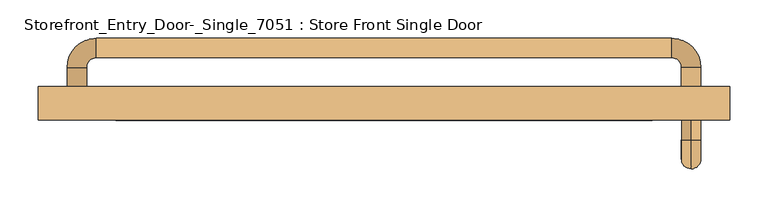
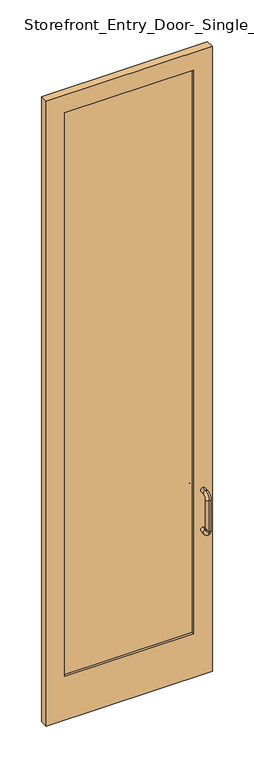
"""IFC4 building model written with IfcOpenShell, lengths in millimetres: door geometry, Storefront_Entry_Door-_Single_7051 : Store Front Single Door."""

import ifcopenshell
import ifcopenshell.guid

model = None  # the IFC model being written
_history = None  # IfcOwnerHistory: only IFC2X3 demands one
_inside = {}  # id of a spatial element -> (the spatial element, [elements in it])
_under = {}  # id of a project, library or spatial element -> (it, [spatial elements below it])
_declared = {}  # id of a project -> (the project, [libraries it declares])
_typed = {}  # id of a type object -> (the type object, [elements of that type])
_made_of = {}  # id of a material, layer set ... -> (it, [elements and type objects made of it])


def new_model(schema):
    """Start an empty IFC model of exactly this schema.

    Asked for "IFC4X3", IfcOpenShell would pick the latest addendum, in which some entities
    have other attributes; the version numbers below select the first issue.
    IFC2X3 requires an IfcOwnerHistory on every rooted entity: one is made here for all.
    """
    global model, _history
    if schema == "IFC4X3":
        model = ifcopenshell.file(schema_version=(4, 3, 0, 0))
    else:
        model = ifcopenshell.file(schema=schema)
    _inside.clear()
    _under.clear()
    _declared.clear()
    _typed.clear()
    _made_of.clear()
    _history = None
    if model.schema == "IFC2X3":
        org = make("IfcOrganization", Name="unknown")
        user = make(
            "IfcPersonAndOrganization",
            ThePerson=make("IfcPerson", FamilyName="unknown"),
            TheOrganization=org,
        )
        app = make(
            "IfcApplication",
            ApplicationDeveloper=org,
            Version="unknown",
            ApplicationFullName="unknown",
            ApplicationIdentifier="unknown",
        )
        _history = make(
            "IfcOwnerHistory",
            OwningUser=user,
            OwningApplication=app,
            ChangeAction="ADDED",
            CreationDate=0,
        )
    return model


def make(cls, **values):
    """One entity of the class cls with the attributes given. An attribute that is None is left unset."""
    return model.create_entity(
        cls, **{name: value for name, value in values.items() if value is not None}
    )


def rooted(cls, **values):
    """An entity with a GlobalId (a new one), such as an element, a storey or a relation."""
    return make(cls, GlobalId=ifcopenshell.guid.new(), OwnerHistory=_history, **values)


def si_unit(unit_type, name, prefix=None):
    """IfcSIUnit, for example si_unit("LENGTHUNIT", "METRE", prefix="MILLI")."""
    return make("IfcSIUnit", UnitType=unit_type, Prefix=prefix, Name=name)


def assignment(units):
    """IfcUnitAssignment: the units of a project."""
    return None if units is None else make("IfcUnitAssignment", Units=units)


def point(xyz):
    """IfcCartesianPoint."""
    return None if xyz is None else make("IfcCartesianPoint", Coordinates=xyz)


def direction(xyz):
    """IfcDirection."""
    return None if xyz is None else make("IfcDirection", DirectionRatios=xyz)


def frame(location, z_axis=None, x_axis=None):
    """IfcAxis2Placement3D, a coordinate frame: its origin and axes. An axis left out is left unset."""
    return make(
        "IfcAxis2Placement3D",
        Location=point(location),
        Axis=direction(z_axis),
        RefDirection=direction(x_axis),
    )


def origin():
    """The frame at (0, 0, 0) with its axes left unset."""
    return frame((0.0, 0.0, 0.0))


def place(relative_to, where):
    """IfcLocalPlacement: puts the frame where relative to a parent placement (None: the world)."""
    return make(
        "IfcLocalPlacement", PlacementRelTo=relative_to, RelativePlacement=where
    )


def context(
    kind, dimensions, precision=None, world=None, true_north=None, identifier=None
):
    """IfcGeometricRepresentationContext, for example the 3D "Model" context."""
    return make(
        "IfcGeometricRepresentationContext",
        ContextIdentifier=identifier,
        ContextType=kind,
        CoordinateSpaceDimension=dimensions,
        Precision=precision,
        WorldCoordinateSystem=world,
        TrueNorth=true_north,
    )


def project(units=None, contexts=None):
    """IfcProject with its units and contexts."""
    return rooted(
        "IfcProject",
        Name="project",
        RepresentationContexts=contexts,
        UnitsInContext=assignment(units),
    )


def spatial(cls, under=None, at=None, **own):
    """A site, building, storey or space (cls), placed at a placement, below another one or the project."""
    s = rooted(cls, ObjectPlacement=at, **own)
    if under is not None:
        _under.setdefault(under.id(), (under, []))[1].append(s)
    return s


def polyline(points):
    """IfcPolyline through the points."""
    return make("IfcPolyline", Points=[point(p) for p in points])


def circle_curve(where, radius):
    """IfcCircle in the frame where."""
    return make("IfcCircle", Position=where, Radius=radius)


def ellipse_curve(where, semi_axis1, semi_axis2):
    """IfcEllipse in the frame where."""
    return make(
        "IfcEllipse", Position=where, SemiAxis1=semi_axis1, SemiAxis2=semi_axis2
    )


def trimmed(basis, trim1, trim2, sense, master):
    """IfcTrimmedCurve: the piece of a basis curve between two trims."""
    return make(
        "IfcTrimmedCurve",
        BasisCurve=basis,
        Trim1=trim1,
        Trim2=trim2,
        SenseAgreement=sense,
        MasterRepresentation=master,
    )


def outline(outer, holes=None, kind="AREA"):
    """IfcArbitraryClosedProfileDef: a profile drawn as a closed curve; with holes, ...WithVoids."""
    if holes is None:
        return make("IfcArbitraryClosedProfileDef", ProfileType=kind, OuterCurve=outer)
    return make(
        "IfcArbitraryProfileDefWithVoids",
        ProfileType=kind,
        OuterCurve=outer,
        InnerCurves=holes,
    )


def extrude(swept, where, along, depth):
    """IfcExtrudedAreaSolid: the profile swept, set in the frame where, extruded along a direction by depth."""
    return make(
        "IfcExtrudedAreaSolid",
        SweptArea=swept,
        Position=where,
        ExtrudedDirection=direction(along),
        Depth=depth,
    )


def shape(context_of_items, identifier, shape_type, items):
    """IfcShapeRepresentation: the items that make up one representation, for example the "Body"."""
    return make(
        "IfcShapeRepresentation",
        ContextOfItems=context_of_items,
        RepresentationIdentifier=identifier,
        RepresentationType=shape_type,
        Items=items,
    )


def source(mapping_origin, context_of_items, identifier, shape_type, items):
    """IfcRepresentationMap: a shape defined once, which mapped items show again and again."""
    return make(
        "IfcRepresentationMap",
        MappingOrigin=mapping_origin,
        MappedRepresentation=shape(context_of_items, identifier, shape_type, items),
    )


def transform(
    local_origin,
    x_axis=None,
    y_axis=None,
    z_axis=None,
    scale=None,
    scale2=None,
    scale3=None,
    uniform=True,
):
    """IfcCartesianTransformationOperator3D, or its non-uniform kind. x_axis, y_axis, z_axis: its Axis1, 2, 3."""
    if uniform:
        return make(
            "IfcCartesianTransformationOperator3D",
            Axis1=direction(x_axis),
            Axis2=direction(y_axis),
            LocalOrigin=point(local_origin),
            Scale=scale,
            Axis3=direction(z_axis),
        )
    return make(
        "IfcCartesianTransformationOperator3DnonUniform",
        Axis1=direction(x_axis),
        Axis2=direction(y_axis),
        LocalOrigin=point(local_origin),
        Scale=scale,
        Axis3=direction(z_axis),
        Scale2=scale2,
        Scale3=scale3,
    )


def mapped(mapping_source, mapping_target):
    """IfcMappedItem: shows the shape of a source again, moved by a transform."""
    return make(
        "IfcMappedItem", MappingSource=mapping_source, MappingTarget=mapping_target
    )


def made_of(thing, what):
    """Note that an element or type object is made of a material, layer set ...; save() writes the relation."""
    if what is not None:
        _made_of.setdefault(what.id(), (what, []))[1].append(thing)
    return thing


def element(
    cls,
    number,
    at=None,
    inside=None,
    cuts=None,
    type_object=None,
    material=None,
    context=None,
    identifier="Body",
    shape_type=None,
    held_by="IfcProductDefinitionShape",
    body=None,
    shapes=None,
    **own,
):
    """One element of the class cls, such as IfcWall. Its Tag is "e" and its number.

    at: its placement. inside: the storey or other place that contains it. cuts: it is an
    opening in that element (IfcRelVoidsElement). A single representation is given by context,
    identifier, shape_type and body (its items); several are given by shapes. held_by: the class
    of the entity that holds the representations. save() writes the other relations.
    """
    e = rooted(cls, Tag="e%d" % number, ObjectPlacement=at, **own)
    if body is not None:
        shapes = [shape(context, identifier, shape_type, body)]
    if shapes is not None:
        e.Representation = make(held_by, Representations=shapes)
    if inside is not None:
        _inside.setdefault(inside.id(), (inside, []))[1].append(e)
    if cuts is not None:
        rooted(
            "IfcRelVoidsElement", RelatingBuildingElement=cuts, RelatedOpeningElement=e
        )
    if type_object is not None:
        _typed.setdefault(type_object.id(), (type_object, []))[1].append(e)
    return made_of(e, material)


def aggregate(whole, parts):
    """IfcRelAggregates: a whole, such as a stair, and the parts it consists of."""
    return rooted("IfcRelAggregates", RelatingObject=whole, RelatedObjects=parts)


def save(model, path):
    """Write the relations noted so far, then the file.

    IfcRelAggregates (storeys below a building ...), IfcRelContainedInSpatialStructure (elements
    in a storey), IfcRelDefinesByType, IfcRelAssociatesMaterial and IfcRelDeclares: one each for
    every whole, place, type object, material and project.
    """
    for whole, parts in _under.values():
        aggregate(whole, parts)
    for where, things in _inside.values():
        rooted(
            "IfcRelContainedInSpatialStructure",
            RelatedElements=things,
            RelatingStructure=where,
        )
    for kind, things in _typed.values():
        rooted("IfcRelDefinesByType", RelatedObjects=things, RelatingType=kind)
    for what, things in _made_of.values():
        rooted("IfcRelAssociatesMaterial", RelatedObjects=things, RelatingMaterial=what)
    for by, libraries in _declared.values():
        rooted("IfcRelDeclares", RelatingContext=by, RelatedDefinitions=libraries)
    model.write(path)


def plane_surface(at):
    """IfcPlane: the flat surface through the origin of the frame at, square to its z axis."""
    return make("IfcPlane", Position=at)


def cylinder_surface(at, radius):
    """IfcCylindricalSurface: all points at the distance radius from the z axis of the frame at."""
    return make("IfcCylindricalSurface", Position=at, Radius=radius)


def revolved_surface(curve, axis_point, axis_direction):
    """IfcSurfaceOfRevolution: the curve turned about the line through axis_point along axis_direction."""
    return make(
        "IfcSurfaceOfRevolution",
        SweptCurve=make("IfcArbitraryOpenProfileDef", ProfileType="CURVE", Curve=curve),
        AxisPosition=make("IfcAxis1Placement", Location=point(axis_point), Axis=direction(axis_direction)),
    )


def advanced_brep(points, edges, surfaces, faces):
    """IfcAdvancedBrep: a solid bounded by faces that lie on surfaces and meet in shared edges.

    An edge is (start, end): straight between two places in points (the first is 0);
    or (start, end, curve); or (start, end, curve, False) where it runs against its curve.
    A face is (place in surfaces, loops), or (place, loops, False) where it looks against
    its surface's normal. A loop lists edges by number (the first is 1), with a minus sign
    where the edge is run from its end to its start. The first loop is the outer one.
    """
    corners = [point(p) for p in points]
    vertices = [make("IfcVertexPoint", VertexGeometry=c) for c in corners]
    made = []
    for start, end, *more in edges:
        made.append(
            make(
                "IfcEdgeCurve",
                EdgeStart=vertices[start],
                EdgeEnd=vertices[end],
                EdgeGeometry=more[0] if more else make("IfcPolyline", Points=[corners[start], corners[end]]),
                SameSense=more[1] if len(more) > 1 else True,
            )
        )
    hull = []
    for where, loops, *sense in faces:
        bounds = []
        for j, loop in enumerate(loops):
            ring = [make("IfcOrientedEdge", EdgeElement=made[abs(k) - 1], Orientation=k > 0) for k in loop]
            bounds.append(
                make(
                    "IfcFaceOuterBound" if j == 0 else "IfcFaceBound",
                    Bound=make("IfcEdgeLoop", EdgeList=ring),
                    Orientation=True,
                )
            )
        hull.append(make("IfcAdvancedFace", Bounds=bounds, FaceSurface=surfaces[where], SameSense=sense[0] if sense else True))
    return make("IfcAdvancedBrep", Outer=make("IfcClosedShell", CfsFaces=hull))


def storefront_entry_door_single_7051_store_front_single_door_77dde46e(model_context):
    return source(origin(), model_context, "Body", "SolidModel", [
        advanced_brep(
        [(402.7714285, -50.8, 1054.1), (402.7714285, -50.8, 1079.5), (402.7714285, -76.2, 1079.5), (402.7714285, -76.2, 1054.1), (402.7714285, -114.3, 1041.4), (402.7714285, -88.9, 1041.4), (402.7714285, -114.3, 863.6), (402.7714285, -88.9, 863.6), (402.7714285, -76.2, 825.5), (402.7714285, -76.2, 850.9), (402.7714285, -50.8, 850.9), (402.7714285, -50.8, 825.5)],
        [
            (0, 1, circle_curve(frame((402.7714285, -50.8, 1066.8), z_axis=(0.0, 1.0, 0.0), x_axis=(0.0, 0.0, 1.0)), 12.7)),
            (1, 0, circle_curve(frame((402.7714285, -50.8, 1066.8), z_axis=(0.0, 1.0, 0.0), x_axis=(0.0, 0.0, 1.0)), 12.7)),
            (1, 2),
            (2, 3, circle_curve(frame((402.7714285, -76.2, 1066.8), z_axis=(0.0, 1.0, 0.0), x_axis=(0.0, 0.0, 1.0)), 12.7)),
            (3, 0),
            (3, 2, circle_curve(frame((402.7714285, -76.2, 1066.8), z_axis=(0.0, 1.0, 0.0), x_axis=(0.0, 0.0, 1.0)), 12.7)),
            (4, 5, circle_curve(frame((402.7714285, -101.6, 1041.4), z_axis=(0.0, 0.0, 1.0), x_axis=(0.0, -1.0, 0.0)), 12.7)),
            (5, 3, circle_curve(frame((402.7714285, -76.2, 1041.4), z_axis=(-1.0, 0.0, 0.0), x_axis=(0.0, 0.0, 1.0)), 12.7)),
            (2, 4, circle_curve(frame((402.7714285, -76.2, 1041.4), z_axis=(1.0, 0.0, 0.0), x_axis=(0.0, 0.0, 1.0)), 38.1)),
            (5, 4, circle_curve(frame((402.7714285, -101.6, 1041.4), z_axis=(0.0, 0.0, 1.0), x_axis=(0.0, -1.0, 0.0)), 12.7)),
            (4, 6),
            (6, 7, circle_curve(frame((402.7714285, -101.6, 863.6), z_axis=(0.0, 0.0, 1.0), x_axis=(0.0, -1.0, 0.0)), 12.7)),
            (7, 5),
            (7, 6, circle_curve(frame((402.7714285, -101.6, 863.6), z_axis=(0.0, 0.0, 1.0), x_axis=(0.0, -1.0, 0.0)), 12.7)),
            (8, 9, circle_curve(frame((402.7714285, -76.2, 838.2), z_axis=(0.0, -1.0, 0.0), x_axis=(0.0, 0.0, -1.0)), 12.7)),
            (9, 7, circle_curve(frame((402.7714285, -76.2, 863.6), z_axis=(-1.0, 0.0, 0.0), x_axis=(0.0, -1.0, 0.0)), 12.7)),
            (6, 8, circle_curve(frame((402.7714285, -76.2, 863.6), z_axis=(1.0, 0.0, 0.0), x_axis=(0.0, -1.0, 0.0)), 38.1)),
            (9, 8, circle_curve(frame((402.7714285, -76.2, 838.2), z_axis=(0.0, -1.0, 0.0), x_axis=(0.0, 0.0, -1.0)), 12.7)),
            (10, 11, circle_curve(frame((402.7714285, -50.8, 838.2), z_axis=(0.0, 1.0, 0.0), x_axis=(0.0, 0.0, -1.0)), 12.7)),
            (11, 10, circle_curve(frame((402.7714285, -50.8, 838.2), z_axis=(0.0, 1.0, 0.0), x_axis=(0.0, 0.0, -1.0)), 12.7)),
            (8, 11),
            (10, 9),
        ],
        [
            plane_surface(frame((402.7714285, -50.8, 1066.8), z_axis=(0.0, 1.0, 0.0), x_axis=(1.0, 0.0, 0.0))),
            cylinder_surface(frame((402.7714285, -50.8, 1066.8), z_axis=(0.0, 1.0, 0.0), x_axis=(0.0, 0.0, 1.0)), 12.7),
            revolved_surface(trimmed(ellipse_curve(frame((402.7714285, -76.2, 1066.8), z_axis=(0.0, -1.0, 0.0), x_axis=(0.0, 0.0, 1.0)), 12.7, 12.7), [point((402.7714285, -76.2, 1054.1))], [point((402.7714285, -76.2, 1079.5))], True, "CARTESIAN"), (402.7714285, -76.2, 1041.4), (-1.0, 0.0, 0.0)),
            revolved_surface(trimmed(ellipse_curve(frame((402.7714285, -76.2, 1066.8), z_axis=(0.0, -1.0, 0.0), x_axis=(0.0, 0.0, 1.0)), 12.7, 12.7), [point((402.7714285, -76.2, 1079.5))], [point((402.7714285, -76.2, 1054.1))], True, "CARTESIAN"), (402.7714285, -76.2, 1041.4), (-1.0, 0.0, 0.0)),
            cylinder_surface(frame((402.7714285, -101.6, 1041.4), z_axis=(0.0, 0.0, 1.0), x_axis=(0.0, -1.0, 0.0)), 12.7),
            revolved_surface(trimmed(ellipse_curve(frame((402.7714285, -101.6, 863.6), z_axis=(0.0, 0.0, -1.0), x_axis=(0.0, -1.0, 0.0)), 12.7, 12.7), [point((402.7714285, -88.9, 863.6))], [point((402.7714285, -114.3, 863.6))], True, "CARTESIAN"), (402.7714285, -76.2, 863.6), (-1.0, 0.0, 0.0)),
            revolved_surface(trimmed(ellipse_curve(frame((402.7714285, -101.6, 863.6), z_axis=(0.0, 0.0, -1.0), x_axis=(0.0, -1.0, 0.0)), 12.7, 12.7), [point((402.7714285, -114.3, 863.6))], [point((402.7714285, -88.9, 863.6))], True, "CARTESIAN"), (402.7714285, -76.2, 863.6), (-1.0, 0.0, 0.0)),
            plane_surface(frame((402.7714285, -50.8, 838.2), z_axis=(0.0, 1.0, 0.0), x_axis=(1.0, 0.0, 0.0))),
            cylinder_surface(frame((402.7714285, -76.2, 838.2), z_axis=(0.0, -1.0, 0.0), x_axis=(0.0, 0.0, -1.0)), 12.7),
        ],
        [
            (0, [[1, 2]]),
            (1, [[3, 4, 5, -2]]),
            (1, [[-5, 6, -3, -1]]),
            (2, [[7, 8, -4, 9]]),
            (3, [[10, -9, -6, -8]]),
            (4, [[11, 12, 13, -7]]),
            (4, [[-13, 14, -11, -10]]),
            (5, [[15, 16, -12, 17]]),
            (6, [[18, -17, -14, -16]]),
            (7, [[19, 20]]),
            (8, [[21, -19, 22, -15]]),
            (8, [[-22, -20, -21, -18]]),
        ],
    ),
        advanced_brep(
        [(390.0714285, -6.35, 1066.8), (415.4714285, -6.35, 1066.8), (415.4714285, 19.05, 1066.8), (390.0714285, 19.05, 1066.8), (377.3714285, 57.15, 1066.8), (377.3714285, 31.75, 1066.8), (-377.3714285, 57.15, 1066.8), (-377.3714285, 31.75, 1066.8), (-415.4714285, 19.05, 1066.8), (-390.0714285, 19.05, 1066.8), (-390.0714285, -6.35, 1066.8), (-415.4714285, -6.35, 1066.8)],
        [
            (0, 1, circle_curve(frame((402.7714285, -6.35, 1066.8), z_axis=(0.0, -1.0, 0.0), x_axis=(1.0, 0.0, 0.0)), 12.7)),
            (1, 0, circle_curve(frame((402.7714285, -6.35, 1066.8), z_axis=(0.0, -1.0, 0.0), x_axis=(1.0, 0.0, 0.0)), 12.7)),
            (1, 2),
            (2, 3, circle_curve(frame((402.7714285, 19.05, 1066.8), z_axis=(0.0, -1.0, 0.0), x_axis=(1.0, 0.0, 0.0)), 12.7)),
            (3, 0),
            (3, 2, circle_curve(frame((402.7714285, 19.05, 1066.8), z_axis=(0.0, -1.0, 0.0), x_axis=(1.0, 0.0, 0.0)), 12.7)),
            (4, 5, circle_curve(frame((377.3714285, 44.45, 1066.8), z_axis=(1.0, 0.0, 0.0), x_axis=(0.0, 1.0, 0.0)), 12.7)),
            (5, 3, circle_curve(frame((377.3714285, 19.05, 1066.8), z_axis=(0.0, 0.0, -1.0), x_axis=(1.0, 0.0, 0.0)), 12.7)),
            (2, 4, circle_curve(frame((377.3714285, 19.05, 1066.8), z_axis=(0.0, 0.0, 1.0), x_axis=(1.0, 0.0, 0.0)), 38.1)),
            (5, 4, circle_curve(frame((377.3714285, 44.45, 1066.8), z_axis=(1.0, 0.0, 0.0), x_axis=(0.0, 1.0, 0.0)), 12.7)),
            (4, 6),
            (6, 7, circle_curve(frame((-377.3714285, 44.45, 1066.8), z_axis=(1.0, 0.0, 0.0), x_axis=(0.0, 1.0, 0.0)), 12.7)),
            (7, 5),
            (7, 6, circle_curve(frame((-377.3714285, 44.45, 1066.8), z_axis=(1.0, 0.0, 0.0), x_axis=(0.0, 1.0, 0.0)), 12.7)),
            (8, 9, circle_curve(frame((-402.7714285, 19.05, 1066.8), z_axis=(0.0, 1.0, 0.0), x_axis=(-1.0, 0.0, 0.0)), 12.7)),
            (9, 7, circle_curve(frame((-377.3714285, 19.05, 1066.8), z_axis=(0.0, 0.0, -1.0), x_axis=(0.0, 1.0, 0.0)), 12.7)),
            (6, 8, circle_curve(frame((-377.3714285, 19.05, 1066.8), z_axis=(0.0, 0.0, 1.0), x_axis=(0.0, 1.0, 0.0)), 38.1)),
            (9, 8, circle_curve(frame((-402.7714285, 19.05, 1066.8), z_axis=(0.0, 1.0, 0.0), x_axis=(-1.0, 0.0, 0.0)), 12.7)),
            (10, 11, circle_curve(frame((-402.7714285, -6.35, 1066.8), z_axis=(0.0, -1.0, 0.0), x_axis=(-1.0, 0.0, 0.0)), 12.7)),
            (11, 10, circle_curve(frame((-402.7714285, -6.35, 1066.8), z_axis=(0.0, -1.0, 0.0), x_axis=(-1.0, 0.0, 0.0)), 12.7)),
            (8, 11),
            (10, 9),
        ],
        [
            plane_surface(frame((402.7714285, -6.35, 1066.8), z_axis=(0.0, -1.0, 0.0), x_axis=(0.0, 0.0, 1.0))),
            cylinder_surface(frame((402.7714285, -6.35, 1066.8), z_axis=(0.0, -1.0, 0.0), x_axis=(1.0, 0.0, 0.0)), 12.7),
            revolved_surface(trimmed(ellipse_curve(frame((402.7714285, 19.05, 1066.8), z_axis=(0.0, 1.0, 0.0), x_axis=(1.0, 0.0, 0.0)), 12.7, 12.7), [point((390.0714285, 19.05, 1066.8))], [point((415.4714285, 19.05, 1066.8))], True, "CARTESIAN"), (377.3714285, 19.05, 1066.8), (0.0, 0.0, -1.0)),
            revolved_surface(trimmed(ellipse_curve(frame((402.7714285, 19.05, 1066.8), z_axis=(0.0, 1.0, 0.0), x_axis=(1.0, 0.0, 0.0)), 12.7, 12.7), [point((415.4714285, 19.05, 1066.8))], [point((390.0714285, 19.05, 1066.8))], True, "CARTESIAN"), (377.3714285, 19.05, 1066.8), (0.0, 0.0, -1.0)),
            cylinder_surface(frame((377.3714285, 44.45, 1066.8), z_axis=(1.0, 0.0, 0.0), x_axis=(0.0, 1.0, 0.0)), 12.7),
            revolved_surface(trimmed(ellipse_curve(frame((-377.3714285, 44.45, 1066.8), z_axis=(-1.0, 0.0, 0.0), x_axis=(0.0, 1.0, 0.0)), 12.7, 12.7), [point((-377.3714285, 31.75, 1066.8))], [point((-377.3714285, 57.15, 1066.8))], True, "CARTESIAN"), (-377.3714285, 19.05, 1066.8), (0.0, 0.0, -1.0)),
            revolved_surface(trimmed(ellipse_curve(frame((-377.3714285, 44.45, 1066.8), z_axis=(-1.0, 0.0, 0.0), x_axis=(0.0, 1.0, 0.0)), 12.7, 12.7), [point((-377.3714285, 57.15, 1066.8))], [point((-377.3714285, 31.75, 1066.8))], True, "CARTESIAN"), (-377.3714285, 19.05, 1066.8), (0.0, 0.0, -1.0)),
            plane_surface(frame((-402.7714285, -6.35, 1066.8), z_axis=(0.0, -1.0, 0.0), x_axis=(0.0, 0.0, 1.0))),
            cylinder_surface(frame((-402.7714285, 19.05, 1066.8), z_axis=(0.0, 1.0, 0.0), x_axis=(-1.0, 0.0, 0.0)), 12.7),
        ],
        [
            (0, [[1, 2]]),
            (1, [[3, 4, 5, -2]]),
            (1, [[-5, 6, -3, -1]]),
            (2, [[7, 8, -4, 9]]),
            (3, [[10, -9, -6, -8]]),
            (4, [[11, 12, 13, -7]]),
            (4, [[-13, 14, -11, -10]]),
            (5, [[15, 16, -12, 17]]),
            (6, [[18, -17, -14, -16]]),
            (7, [[19, 20]]),
            (8, [[21, -19, 22, -15]]),
            (8, [[-22, -20, -21, -18]]),
        ],
    ),
        extrude(outline(polyline([(351.9714285, -19.05), (351.9714285, -38.1), (-351.9714285, -38.1), (-351.9714285, -19.05), (351.9714285, -19.05)])), frame((0.0, 0.0, 254.0), z_axis=(0.0, 0.0, 1.0), x_axis=(1.0, 0.0, 0.0)), (0.0, 0.0, 1.0), 3251.2),
        extrude(outline(polyline([(3606.8, 453.5714285), (3606.8, -453.5714285), (0.0, -453.5714285), (0.0, 453.5714285), (3606.8, 453.5714285)]), holes=[polyline([(3505.2, -351.9714285), (3505.2, 351.9714285), (254.0, 351.9714285), (254.0, -351.9714285), (3505.2, -351.9714285)])]), frame((0.0, -50.8, 0.0), z_axis=(0.0, 1.0, 0.0), x_axis=(0.0, 0.0, 1.0)), (0.0, 0.0, 1.0), 44.45),
    ])


if __name__ == "__main__":
    model = new_model("IFC4")
    model_context = context("Model", 3, world=origin())
    ifc_project = project(units=[si_unit("LENGTHUNIT", "METRE", prefix="MILLI")], contexts=[model_context])
    site = spatial("IfcSite", under=ifc_project)
    building = spatial("IfcBuilding", under=site)
    placement = place(None, origin())
    storefront_entry_door_single_7051_store_front_single_door_shape = storefront_entry_door_single_7051_store_front_single_door_77dde46e(model_context)
    element("IfcDoor", 1, ObjectType="Storefront_Entry_Door-_Single_7051 : Store Front Single Door", at=placement, inside=building, context=model_context, shape_type="MappedRepresentation", body=[
        mapped(storefront_entry_door_single_7051_store_front_single_door_shape, transform((0.0, 0.0, 0.0), x_axis=(1.0, 0.0, 0.0), y_axis=(0.0, 1.0, 0.0), z_axis=(0.0, 0.0, 1.0))),
    ])
    save(model, "model.ifc")

# Revit data of these elements
# Type "Storefront_Entry_Door-_Single_7051 : Store Front Single Door"
#   Type Mark = "19"
#   Assembly Code = "B2030110"
#   Analytic Construction = "<None>"
#   Top Rail = 0' - 4"
#   Side Rail = 0' - 4"
#   Reporting Width [instance default] = 4' - 2"
#   Rail Height AFF = 3' - 6"
#   Offset = 0' - 2"
#   Door Width [instance default] = 4' - 2"
#   Bottom Rail Width = 0' - 10"
#   Material = PAINTED STEEL C CHANNEL
#   Glazing Material = BUTT GLAZED STOREFRONT WITH VERTICAL MULLION
#   Function = (empty or 0)
# Element 1 (IfcDoor, "Storefront_Entry_Door-_Single_7051 : Store Front Single Door")
#   Reporting Width = 2' - 11.71429"
#   Door Width = 2' - 11.71429"
#   Materials on its faces: "PAINTED STEEL C CHANNEL", "BUTT GLAZED STOREFRONT WITH VERTICAL MULLION"
# Materials
#   "PAINTED STEEL C CHANNEL": class "Generic", colour RGB 88 62 61, transparency 0, Cost = 0
#   "BUTT GLAZED STOREFRONT WITH VERTICAL MULLION": class "Glass", colour RGB 236 240 239, transparency 0.39, Description = "Soda Lime Glass", Cost = 0
